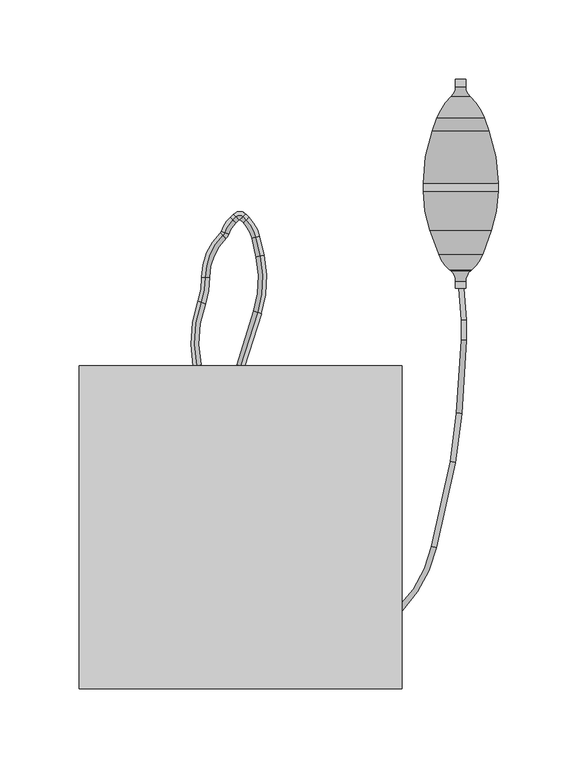
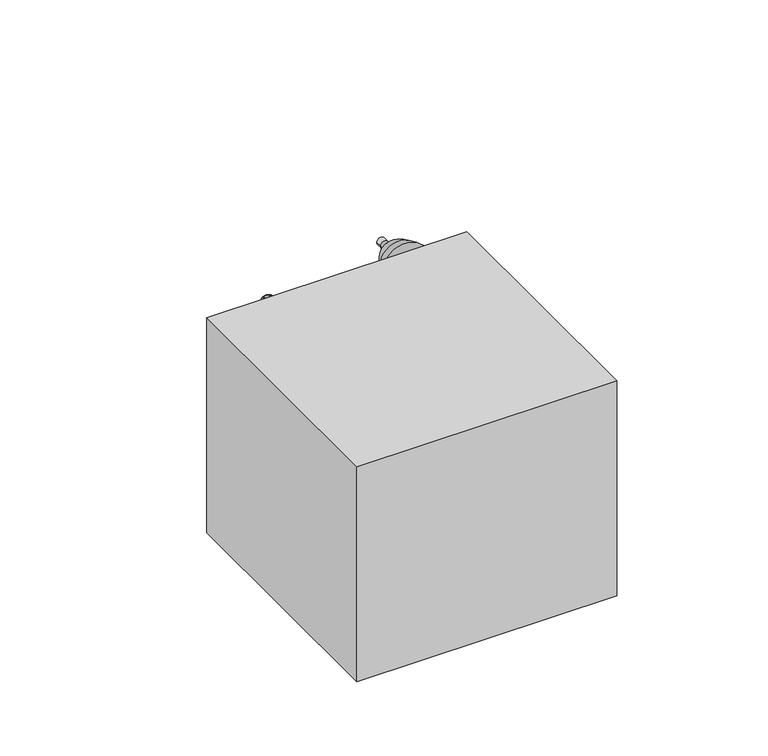
"""IFC4 building model written with IfcOpenShell, lengths in millimetres: proxy geometry, M4100 - Sphygmomanometer, Aneroid, Wall-Mounted : M4100 - Sphygmomanometer, Aneroid, Wall-Mounted."""

from ifc_helpers import new_model, si_unit, point, frame, frame_2d, origin, origin_with_axes, place, context, project, spatial, polyline, circle_curve, ellipse_curve, trimmed, segment, composite_curve, outline, extrude, source, transform, mapped, element, save
from ifc_brep_helpers import plane_surface, cylinder_surface, revolved_surface, extruded_surface, advanced_brep


def specialty_equipment_1a292596(model_context):
    return source(origin(), model_context, "Body", "SolidModel", [
        advanced_brep(
        [(0.0, 0.0, 93.3890108), (0.0, 0.0, 103.4609892), (10.60129, 33.4899695, 103.4609892), (10.60129, 33.4899695, 93.3890108), (12.1452256, 68.8519095, 103.4609892), (12.1452256, 68.8519095, 93.3890108), (9.4902706, 80.7634297, 103.4609892), (9.4902706, 80.7634297, 93.3890108), (3.5257448, 91.6206606, 103.4609892), (3.5257448, 91.6206606, 93.3890108), (1.489236, 93.6571694, 103.4609892), (1.489236, 93.6571694, 93.3890108), (-2.7411458, 93.6571694, 103.4609892), (-2.7411458, 93.6571694, 93.3890108), (-4.6658712, 91.732444, 103.4609892), (-4.6658712, 91.732444, 93.3890108), (-9.7582734, 83.8141156, 103.4609892), (-9.7582734, 83.8141156, 93.3890108), (-10.9708227, 81.9675873, 103.4609892), (-10.9708227, 81.9675873, 93.3890108), (-21.9594666, 55.7504476, 103.4609892), (-21.9594666, 55.7504476, 93.3890108), (-24.5939327, 39.9510684, 103.4609892), (-24.5939327, 39.9510684, 93.3890108), (-27.3580457, 0.1117834, 93.3890108), (-27.3580457, 0.1117834, 103.4609892)],
        [
            (0, 1, ellipse_curve(frame((0.0, 0.0, 98.425), z_axis=(-0.30179165133573443, -0.9533739031377199, 0.0), x_axis=(0.0, 0.0, 1.0)), 5.0359892, 2.5179946)),
            (1, 0, ellipse_curve(frame((0.0, 0.0, 98.425), z_axis=(-0.30179165133573443, -0.9533739031377199, 0.0), x_axis=(0.0, 0.0, 1.0)), 5.0359892, 2.5179946)),
            (1, 2),
            (2, 3, ellipse_curve(frame((10.60129, 33.4899695, 98.425), z_axis=(-0.3017916513357344, -0.9533739031377201, 0.0), x_axis=(0.0, 0.0, 1.0)), 5.0359892, 2.5179946)),
            (3, 0),
            (3, 2, ellipse_curve(frame((10.60129, 33.4899695, 98.425), z_axis=(-0.3017916513357344, -0.9533739031377201, 0.0), x_axis=(0.0, 0.0, 1.0)), 5.0359892, 2.5179946)),
            (4, 5, ellipse_curve(frame((12.1452256, 68.8519095, 98.425), z_axis=(0.21755123234481033, -0.9760489031320381, 0.0), x_axis=(0.0, 0.0, 1.0)), 5.0359892, 2.5179946)),
            (5, 3, circle_curve(frame((-54.3137244, 54.0388951, 93.3890108), z_axis=(0.0, 0.0, -1.0), x_axis=(0.9533739031377199, -0.3017916513357344, 0.0)), 68.0897748)),
            (2, 4, circle_curve(frame((-54.3137244, 54.0388951, 103.4609892), z_axis=(0.0, 0.0, 1.0), x_axis=(0.9533739031377199, -0.3017916513357344, 0.0)), 68.0897748)),
            (5, 4, ellipse_curve(frame((12.1452256, 68.8519095, 98.425), z_axis=(0.21755123234481044, -0.9760489031320381, 0.0), x_axis=(0.0, 0.0, 1.0)), 5.0359892, 2.5179946)),
            (4, 6),
            (6, 7, ellipse_curve(frame((9.4902706, 80.7634297, 98.425), z_axis=(0.21755123234481058, -0.9760489031320381, 0.0), x_axis=(0.0, 0.0, 1.0)), 5.0359892, 2.5179946)),
            (7, 5),
            (7, 6, ellipse_curve(frame((9.4902706, 80.7634297, 98.425), z_axis=(0.21755123234481058, -0.9760489031320381, 0.0), x_axis=(0.0, 0.0, 1.0)), 5.0359892, 2.5179946)),
            (8, 9, ellipse_curve(frame((3.5257448, 91.6206606, 98.425), z_axis=(0.7071067811865478, -0.7071067811865472, 0.0), x_axis=(0.0, 0.0, 1.0)), 5.0359892, 2.5179946)),
            (9, 7, circle_curve(frame((-12.1562786, 75.9386371, 93.3890108), z_axis=(0.0, 0.0, -1.0), x_axis=(0.9760489031320378, 0.21755123234481052, 0.0)), 22.1777302)),
            (6, 8, circle_curve(frame((-12.1562786, 75.9386371, 103.4609892), z_axis=(0.0, 0.0, 1.0), x_axis=(0.9760489031320378, 0.21755123234481052, 0.0)), 22.1777302)),
            (9, 8, ellipse_curve(frame((3.5257448, 91.6206606, 98.425), z_axis=(0.7071067811865477, -0.7071067811865474, 0.0), x_axis=(0.0, 0.0, 1.0)), 5.0359892, 2.5179946)),
            (8, 10),
            (10, 11, ellipse_curve(frame((1.489236, 93.6571694, 98.425), z_axis=(0.7071067811865424, -0.7071067811865528, 0.0), x_axis=(0.0, 0.0, 1.0)), 5.0359892, 2.5179946)),
            (11, 9),
            (11, 10, ellipse_curve(frame((1.489236, 93.6571694, 98.425), z_axis=(0.7071067811865424, -0.7071067811865528, 0.0), x_axis=(0.0, 0.0, 1.0)), 5.0359892, 2.5179946)),
            (12, 13, ellipse_curve(frame((-2.7411458, 93.6571694, 98.425), z_axis=(0.7071067811865475, 0.7071067811865477, 0.0), x_axis=(0.0, 0.0, 1.0)), 5.0359892, 2.5179946)),
            (13, 11, circle_curve(frame((-0.6259549, 91.5419785, 93.3890108), z_axis=(0.0, 0.0, -1.0), x_axis=(0.7071067811865528, 0.7071067811865424, 0.0)), 2.9913317)),
            (10, 12, circle_curve(frame((-0.6259549, 91.5419785, 103.4609892), z_axis=(0.0, 0.0, 1.0), x_axis=(0.7071067811865528, 0.7071067811865424, 0.0)), 2.9913317)),
            (13, 12, ellipse_curve(frame((-2.7411458, 93.6571694, 98.425), z_axis=(0.7071067811865426, 0.7071067811865526, 0.0), x_axis=(0.0, 0.0, 1.0)), 5.0359892, 2.5179946)),
            (12, 14),
            (14, 15, ellipse_curve(frame((-4.6658712, 91.732444, 98.425), z_axis=(0.7071067811865434, 0.7071067811865517, 0.0), x_axis=(0.0, 0.0, 1.0)), 5.0359892, 2.5179946)),
            (15, 13),
            (15, 14, ellipse_curve(frame((-4.6658712, 91.732444, 98.425), z_axis=(0.7071067811865434, 0.7071067811865517, 0.0), x_axis=(0.0, 0.0, 1.0)), 5.0359892, 2.5179946)),
            (16, 17, ellipse_curve(frame((-9.7582734, 83.8141156, 98.425), z_axis=(0.35006716200403615, 0.9367246031179283, 0.0), x_axis=(0.0, 0.0, 1.0)), 5.0359892, 2.5179946)),
            (17, 15, circle_curve(frame((11.0161522, 76.0504205, 93.3890108), z_axis=(0.0, 0.0, -1.0), x_axis=(-0.7071067811865517, 0.7071067811865434, 0.0)), 22.1777302)),
            (14, 16, circle_curve(frame((11.0161522, 76.0504205, 103.4609892), z_axis=(0.0, 0.0, 1.0), x_axis=(-0.7071067811865517, 0.7071067811865434, 0.0)), 22.1777302)),
            (17, 16, ellipse_curve(frame((-9.7582734, 83.8141156, 98.425), z_axis=(0.35006716200403576, 0.9367246031179283, 0.0), x_axis=(0.0, 0.0, 1.0)), 5.0359892, 2.5179946)),
            (18, 19, ellipse_curve(frame((-10.9708227, 81.9675873, 98.425), z_axis=(0.7204486556395683, 0.6935082801143322, 0.0), x_axis=(0.0, 0.0, 1.0)), 5.0359892, 2.5179946)),
            (19, 17, circle_curve(frame((-14.4282922, 85.5593673, 93.3890108), z_axis=(0.0, 0.0, 1.0), x_axis=(0.9367246031179312, -0.3500671620040279, 0.0)), 4.9854768)),
            (16, 18, circle_curve(frame((-14.4282922, 85.5593673, 103.4609892), z_axis=(0.0, 0.0, -1.0), x_axis=(0.9367246031179312, -0.3500671620040279, 0.0)), 4.9854768)),
            (19, 18, ellipse_curve(frame((-10.9708227, 81.9675873, 98.425), z_axis=(0.7204486556395688, 0.6935082801143314, 0.0), x_axis=(0.0, 0.0, 1.0)), 5.0359892, 2.5179946)),
            (20, 21, ellipse_curve(frame((-21.9594666, 55.7504476, 98.425), z_axis=(-0.010655908230738531, 0.9999432241981432, 0.0), x_axis=(0.0, 0.0, 1.0)), 5.0359892, 2.5179946)),
            (21, 19, circle_curve(frame((13.8981281, 56.1325645, 93.3890108), z_axis=(0.0, 0.0, -1.0), x_axis=(-0.6935082801143324, 0.7204486556395678, 0.0)), 35.8596307)),
            (18, 20, circle_curve(frame((13.8981281, 56.1325645, 103.4609892), z_axis=(0.0, 0.0, 1.0), x_axis=(-0.6935082801143324, 0.7204486556395678, 0.0)), 35.8596307)),
            (21, 20, ellipse_curve(frame((-21.9594666, 55.7504476, 98.425), z_axis=(-0.010655908230738309, 0.9999432241981432, 0.0), x_axis=(0.0, 0.0, 1.0)), 5.0359892, 2.5179946)),
            (22, 23, ellipse_curve(frame((-24.5939327, 39.9510684, 98.425), z_axis=(0.33452931398523156, 0.9423853447950952, 0.0), x_axis=(0.0, 0.0, 1.0)), 5.0359892, 2.5179946)),
            (23, 21, circle_curve(frame((-67.7275968, 55.2627189, 93.3890108), z_axis=(0.0, 0.0, 1.0), x_axis=(0.9999432241981431, 0.010655908230754234, 0.0)), 45.7707289)),
            (20, 22, circle_curve(frame((-67.7275968, 55.2627189, 103.4609892), z_axis=(0.0, 0.0, -1.0), x_axis=(0.9999432241981431, 0.010655908230754234, 0.0)), 45.7707289)),
            (23, 22, ellipse_curve(frame((-24.5939327, 39.9510684, 98.425), z_axis=(0.3345293139852315, 0.9423853447950952, 0.0), x_axis=(0.0, 0.0, 1.0)), 5.0359892, 2.5179946)),
            (24, 25, ellipse_curve(frame((-27.3580457, 0.1117834, 98.425), z_axis=(0.2011821163330489, -0.9795538556239548, 0.0), x_axis=(0.0, 0.0, 1.0)), 5.0359892, 2.5179946)),
            (25, 24, ellipse_curve(frame((-27.3580457, 0.1117834, 98.425), z_axis=(0.2011821163330489, -0.9795538556239548, 0.0), x_axis=(0.0, 0.0, 1.0)), 5.0359892, 2.5179946)),
            (24, 23, circle_curve(frame((45.4884963, 15.0731063, 93.3890108), z_axis=(0.0, 0.0, -1.0), x_axis=(-0.9423853447950952, 0.33452931398523145, 0.0)), 74.3670617)),
            (22, 25, circle_curve(frame((45.4884963, 15.0731063, 103.4609892), z_axis=(0.0, 0.0, 1.0), x_axis=(-0.9423853447950952, 0.33452931398523145, 0.0)), 74.3670617)),
        ],
        [
            plane_surface(frame((0.0, 0.0, 98.425), z_axis=(-0.30179165133573443, -0.9533739031377199, 0.0), x_axis=(0.0, 0.0, 1.0))),
            extruded_surface(trimmed(ellipse_curve(frame((0.0, 0.0, 98.425), z_axis=(0.30179165133573443, 0.9533739031377199, 0.0), x_axis=(0.0, 0.0, 1.0)), 5.0359892, 2.5179946), [point((0.0, 0.0, 93.3890108))], [point((0.0, 0.0, 103.4609892))], True, "CARTESIAN"), (10.60129, 33.4899695, 0.0), 35.1278437535672),
            extruded_surface(trimmed(ellipse_curve(frame((0.0, 0.0, 98.425), z_axis=(0.30179165133573443, 0.9533739031377199, 0.0), x_axis=(0.0, 0.0, 1.0)), 5.0359892, 2.5179946), [point((0.0, 0.0, 103.4609892))], [point((0.0, 0.0, 93.3890108))], True, "CARTESIAN"), (10.60129, 33.4899695, 0.0), 35.1278437535672),
            revolved_surface(trimmed(ellipse_curve(frame((10.60129, 33.4899695, 98.425), z_axis=(0.3017916513357343, 0.9533739031377199, 0.0), x_axis=(0.0, 0.0, 1.0)), 5.0359892, 2.5179946), [point((10.60129, 33.4899695, 93.3890108))], [point((10.60129, 33.4899695, 103.4609892))], True, "CARTESIAN"), (-54.3137244, 54.0388951, 98.425), (0.0, 0.0, -1.0)),
            revolved_surface(trimmed(ellipse_curve(frame((10.60129, 33.4899695, 98.425), z_axis=(0.3017916513357343, 0.9533739031377199, 0.0), x_axis=(0.0, 0.0, 1.0)), 5.0359892, 2.5179946), [point((10.60129, 33.4899695, 103.4609892))], [point((10.60129, 33.4899695, 93.3890108))], True, "CARTESIAN"), (-54.3137244, 54.0388951, 98.425), (0.0, 0.0, -1.0)),
            extruded_surface(trimmed(ellipse_curve(frame((12.1452256, 68.8519095, 98.425), z_axis=(-0.2175512323448103, 0.976048903132038, 0.0), x_axis=(0.0, 0.0, 1.0)), 5.0359892, 2.5179946), [point((12.1452256, 68.8519095, 93.3890108))], [point((12.1452256, 68.8519095, 103.4609892))], True, "CARTESIAN"), (-2.6549549999999993, 11.911520199999998, 0.0), 12.203814957915126),
            extruded_surface(trimmed(ellipse_curve(frame((12.1452256, 68.8519095, 98.425), z_axis=(-0.2175512323448103, 0.976048903132038, 0.0), x_axis=(0.0, 0.0, 1.0)), 5.0359892, 2.5179946), [point((12.1452256, 68.8519095, 103.4609892))], [point((12.1452256, 68.8519095, 93.3890108))], True, "CARTESIAN"), (-2.6549549999999993, 11.911520199999998, 0.0), 12.203814957915126),
            revolved_surface(trimmed(ellipse_curve(frame((9.4902706, 80.7634297, 98.425), z_axis=(-0.21755123234481052, 0.9760489031320378, 0.0), x_axis=(0.0, 0.0, 1.0)), 5.0359892, 2.5179946), [point((9.4902706, 80.7634297, 93.3890108))], [point((9.4902706, 80.7634297, 103.4609892))], True, "CARTESIAN"), (-12.1562786, 75.9386371, 98.425), (0.0, 0.0, -1.0)),
            revolved_surface(trimmed(ellipse_curve(frame((9.4902706, 80.7634297, 98.425), z_axis=(-0.21755123234481052, 0.9760489031320378, 0.0), x_axis=(0.0, 0.0, 1.0)), 5.0359892, 2.5179946), [point((9.4902706, 80.7634297, 103.4609892))], [point((9.4902706, 80.7634297, 93.3890108))], True, "CARTESIAN"), (-12.1562786, 75.9386371, 98.425), (0.0, 0.0, -1.0)),
            extruded_surface(trimmed(ellipse_curve(frame((3.5257448, 91.6206606, 98.425), z_axis=(-0.707106781186548, 0.707106781186547, 0.0), x_axis=(0.0, 0.0, 1.0)), 5.0359892, 2.5179946), [point((3.5257448, 91.6206606, 93.3890108))], [point((3.5257448, 91.6206606, 103.4609892))], True, "CARTESIAN"), (-2.0365088, 2.036508800000007, 0.0), 2.8800583648521623),
            extruded_surface(trimmed(ellipse_curve(frame((3.5257448, 91.6206606, 98.425), z_axis=(-0.707106781186548, 0.707106781186547, 0.0), x_axis=(0.0, 0.0, 1.0)), 5.0359892, 2.5179946), [point((3.5257448, 91.6206606, 103.4609892))], [point((3.5257448, 91.6206606, 93.3890108))], True, "CARTESIAN"), (-2.0365088, 2.036508800000007, 0.0), 2.8800583648521623),
            revolved_surface(trimmed(ellipse_curve(frame((1.489236, 93.6571694, 98.425), z_axis=(-0.7071067811865424, 0.7071067811865528, 0.0), x_axis=(0.0, 0.0, 1.0)), 5.0359892, 2.5179946), [point((1.489236, 93.6571694, 93.3890108))], [point((1.489236, 93.6571694, 103.4609892))], True, "CARTESIAN"), (-0.6259549, 91.5419785, 98.425), (0.0, 0.0, -1.0)),
            revolved_surface(trimmed(ellipse_curve(frame((1.489236, 93.6571694, 98.425), z_axis=(-0.7071067811865424, 0.7071067811865528, 0.0), x_axis=(0.0, 0.0, 1.0)), 5.0359892, 2.5179946), [point((1.489236, 93.6571694, 103.4609892))], [point((1.489236, 93.6571694, 93.3890108))], True, "CARTESIAN"), (-0.6259549, 91.5419785, 98.425), (0.0, 0.0, -1.0)),
            extruded_surface(trimmed(ellipse_curve(frame((-2.7411458, 93.6571694, 98.425), z_axis=(-0.707106781186542, -0.7071067811865531, 0.0), x_axis=(0.0, 0.0, 1.0)), 5.0359892, 2.5179946), [point((-2.7411458, 93.6571694, 93.3890108))], [point((-2.7411458, 93.6571694, 103.4609892))], True, "CARTESIAN"), (-1.9247253999999998, -1.9247253999999998, 0.0), 2.72197276452398),
            extruded_surface(trimmed(ellipse_curve(frame((-2.7411458, 93.6571694, 98.425), z_axis=(-0.707106781186542, -0.7071067811865531, 0.0), x_axis=(0.0, 0.0, 1.0)), 5.0359892, 2.5179946), [point((-2.7411458, 93.6571694, 103.4609892))], [point((-2.7411458, 93.6571694, 93.3890108))], True, "CARTESIAN"), (-1.9247253999999998, -1.9247253999999998, 0.0), 2.72197276452398),
            revolved_surface(trimmed(ellipse_curve(frame((-4.6658712, 91.732444, 98.425), z_axis=(-0.7071067811865434, -0.7071067811865517, 0.0), x_axis=(0.0, 0.0, 1.0)), 5.0359892, 2.5179946), [point((-4.6658712, 91.732444, 93.3890108))], [point((-4.6658712, 91.732444, 103.4609892))], True, "CARTESIAN"), (11.0161522, 76.0504205, 98.425), (0.0, 0.0, -1.0)),
            revolved_surface(trimmed(ellipse_curve(frame((-4.6658712, 91.732444, 98.425), z_axis=(-0.7071067811865434, -0.7071067811865517, 0.0), x_axis=(0.0, 0.0, 1.0)), 5.0359892, 2.5179946), [point((-4.6658712, 91.732444, 103.4609892))], [point((-4.6658712, 91.732444, 93.3890108))], True, "CARTESIAN"), (11.0161522, 76.0504205, 98.425), (0.0, 0.0, -1.0)),
            revolved_surface(trimmed(ellipse_curve(frame((-9.7582734, 83.8141156, 98.425), z_axis=(-0.350067162004028, -0.9367246031179312, 0.0), x_axis=(0.0, 0.0, 1.0)), 5.0359892, 2.5179946), [point((-9.7582734, 83.8141156, 93.3890108))], [point((-9.7582734, 83.8141156, 103.4609892))], True, "CARTESIAN"), (-14.4282922, 85.5593673, 98.425), (0.0, 0.0, 1.0)),
            revolved_surface(trimmed(ellipse_curve(frame((-9.7582734, 83.8141156, 98.425), z_axis=(-0.350067162004028, -0.9367246031179312, 0.0), x_axis=(0.0, 0.0, 1.0)), 5.0359892, 2.5179946), [point((-9.7582734, 83.8141156, 103.4609892))], [point((-9.7582734, 83.8141156, 93.3890108))], True, "CARTESIAN"), (-14.4282922, 85.5593673, 98.425), (0.0, 0.0, 1.0)),
            revolved_surface(trimmed(ellipse_curve(frame((-10.9708227, 81.9675873, 98.425), z_axis=(-0.7204486556395681, -0.6935082801143322, 0.0), x_axis=(0.0, 0.0, 1.0)), 5.0359892, 2.5179946), [point((-10.9708227, 81.9675873, 93.3890108))], [point((-10.9708227, 81.9675873, 103.4609892))], True, "CARTESIAN"), (13.8981281, 56.1325645, 98.425), (0.0, 0.0, -1.0)),
            revolved_surface(trimmed(ellipse_curve(frame((-10.9708227, 81.9675873, 98.425), z_axis=(-0.7204486556395681, -0.6935082801143322, 0.0), x_axis=(0.0, 0.0, 1.0)), 5.0359892, 2.5179946), [point((-10.9708227, 81.9675873, 103.4609892))], [point((-10.9708227, 81.9675873, 93.3890108))], True, "CARTESIAN"), (13.8981281, 56.1325645, 98.425), (0.0, 0.0, -1.0)),
            revolved_surface(trimmed(ellipse_curve(frame((-21.9594666, 55.7504476, 98.425), z_axis=(0.010655908230753961, -0.9999432241981431, 0.0), x_axis=(0.0, 0.0, 1.0)), 5.0359892, 2.5179946), [point((-21.9594666, 55.7504476, 93.3890108))], [point((-21.9594666, 55.7504476, 103.4609892))], True, "CARTESIAN"), (-67.7275968, 55.2627189, 98.425), (0.0, 0.0, 1.0)),
            revolved_surface(trimmed(ellipse_curve(frame((-21.9594666, 55.7504476, 98.425), z_axis=(0.010655908230753961, -0.9999432241981431, 0.0), x_axis=(0.0, 0.0, 1.0)), 5.0359892, 2.5179946), [point((-21.9594666, 55.7504476, 103.4609892))], [point((-21.9594666, 55.7504476, 93.3890108))], True, "CARTESIAN"), (-67.7275968, 55.2627189, 98.425), (0.0, 0.0, 1.0)),
            plane_surface(frame((-27.3580457, 0.1117834, 98.425), z_axis=(0.201182116333049, -0.9795538556239548, 0.0), x_axis=(0.0, 0.0, 1.0))),
            revolved_surface(trimmed(ellipse_curve(frame((-24.5939327, 39.9510684, 98.425), z_axis=(-0.3345293139852318, -0.9423853447950951, 0.0), x_axis=(0.0, 0.0, 1.0)), 5.0359892, 2.5179946), [point((-24.5939327, 39.9510684, 93.3890108))], [point((-24.5939327, 39.9510684, 103.4609892))], True, "CARTESIAN"), (45.4884963, 15.0731063, 98.425), (0.0, 0.0, -1.0)),
            revolved_surface(trimmed(ellipse_curve(frame((-24.5939327, 39.9510684, 98.425), z_axis=(-0.3345293139852318, -0.9423853447950951, 0.0), x_axis=(0.0, 0.0, 1.0)), 5.0359892, 2.5179946), [point((-24.5939327, 39.9510684, 103.4609892))], [point((-24.5939327, 39.9510684, 93.3890108))], True, "CARTESIAN"), (45.4884963, 15.0731063, 98.425), (0.0, 0.0, -1.0)),
        ],
        [
            (0, [[1, 2]]),
            (1, [[3, 4, 5, -2]]),
            (2, [[-5, 6, -3, -1]]),
            (3, [[7, 8, -4, 9]]),
            (4, [[10, -9, -6, -8]]),
            (5, [[11, 12, 13, -7]]),
            (6, [[-13, 14, -11, -10]]),
            (7, [[15, 16, -12, 17]]),
            (8, [[18, -17, -14, -16]]),
            (9, [[19, 20, 21, -15]]),
            (10, [[-21, 22, -19, -18]]),
            (11, [[23, 24, -20, 25]]),
            (12, [[26, -25, -22, -24]]),
            (13, [[27, 28, 29, -23]]),
            (14, [[-29, 30, -27, -26]]),
            (15, [[31, 32, -28, 33]]),
            (16, [[34, -33, -30, -32]]),
            (17, [[35, 36, -31, 37]]),
            (18, [[38, -37, -34, -36]]),
            (19, [[39, 40, -35, 41]]),
            (20, [[42, -41, -38, -40]]),
            (21, [[43, 44, -39, 45]]),
            (22, [[46, -45, -42, -44]]),
            (23, [[47, 48]]),
            (24, [[-47, 49, -43, 50]]),
            (25, [[-48, -50, -46, -49]]),
        ],
    ),
        advanced_brep(
        [(138.1282079, 48.8005767, 47.6946196), (135.3817713, 48.8005767, 47.6946196), (141.8571136, 48.8005767, 47.6946196), (139.110677, 48.8005767, 47.6946196), (138.1282079, 180.1855223, 47.6946196), (139.110677, 180.1855223, 47.6946196), (135.3817713, 180.1855223, 47.6946196), (141.8571136, 180.1855223, 47.6946196), (135.3817713, 175.5632852, 47.6946196), (141.8571136, 175.5632852, 47.6946196), (132.7169258, 169.4696535, 47.6946196), (144.5219592, 169.4696535, 47.6946196), (123.7575473, 155.9951928, 47.6946196), (153.4813376, 155.9951928, 47.6946196), (120.8482177, 148.0018755, 47.6946196), (156.3906672, 148.0018755, 47.6946196), (114.9866942, 114.7595239, 47.6946196), (162.2521907, 114.7595239, 47.6946196), (114.9866942, 109.7483973, 47.6946196), (162.2521907, 109.7483973, 47.6946196), (119.3165907, 85.1923341, 47.6946196), (157.9222942, 85.1923341, 47.6946196), (124.8056359, 70.1113063, 47.6946196), (152.433249, 70.1113063, 47.6946196), (131.6106524, 60.3927356, 47.6946196), (145.6282325, 60.3927356, 47.6946196), (132.2844617, 59.8273424, 47.6946196), (144.9544232, 59.8273424, 47.6946196), (135.3817713, 53.1851407, 47.6946196), (141.8571136, 53.1851407, 47.6946196)],
        [
            (0, 1),
            (1, 2, circle_curve(frame((138.6194425, 48.8005767, 47.6946196), z_axis=(0.0, -1.0, 0.0), x_axis=(1.0, 0.0, 0.0)), 3.2376712)),
            (2, 3),
            (3, 0, circle_curve(frame((138.6194425, 48.8005767, 47.6946196), z_axis=(0.0, 1.0, 0.0), x_axis=(1.0, 0.0, 0.0)), 0.4912345)),
            (2, 1, circle_curve(frame((138.6194425, 48.8005767, 47.6946196), z_axis=(0.0, -1.0, 0.0), x_axis=(1.0, 0.0, 0.0)), 3.2376712)),
            (0, 3, circle_curve(frame((138.6194425, 48.8005767, 47.6946196), z_axis=(0.0, 1.0, 0.0), x_axis=(1.0, 0.0, 0.0)), 0.4912345)),
            (4, 0),
            (3, 5),
            (5, 4, circle_curve(frame((138.6194425, 180.1855223, 47.6946196), z_axis=(0.0, 1.0, 0.0), x_axis=(1.0, 0.0, 0.0)), 0.4912345)),
            (4, 5, circle_curve(frame((138.6194425, 180.1855223, 47.6946196), z_axis=(0.0, 1.0, 0.0), x_axis=(1.0, 0.0, 0.0)), 0.4912345)),
            (6, 4),
            (5, 7),
            (7, 6, circle_curve(frame((138.6194425, 180.1855223, 47.6946196), z_axis=(0.0, 1.0, 0.0), x_axis=(1.0, 0.0, 0.0)), 3.2376712)),
            (6, 7, circle_curve(frame((138.6194425, 180.1855223, 47.6946196), z_axis=(0.0, 1.0, 0.0), x_axis=(1.0, 0.0, 0.0)), 3.2376712)),
            (8, 6),
            (7, 9),
            (9, 8, circle_curve(frame((138.6194425, 175.5632852, 47.6946196), z_axis=(0.0, 1.0, 0.0), x_axis=(1.0, 0.0, 0.0)), 3.2376712)),
            (8, 9, circle_curve(frame((138.6194425, 175.5632852, 47.6946196), z_axis=(0.0, 1.0, 0.0), x_axis=(1.0, 0.0, 0.0)), 3.2376712)),
            (10, 8, circle_curve(frame((127.0822753, 175.5632852, 47.6946196), z_axis=(0.0, 0.0, 1.0), x_axis=(-1.0, 0.0, 0.0)), 8.299496)),
            (9, 11, circle_curve(frame((150.1566096, 175.5632852, 47.6946196), z_axis=(0.0, 0.0, 1.0), x_axis=(1.0, 0.0, 0.0)), 8.299496)),
            (11, 10, circle_curve(frame((138.6194425, 169.4696535, 47.6946196), z_axis=(0.0, 1.0, 0.0), x_axis=(1.0, 0.0, 0.0)), 5.9025167)),
            (10, 11, circle_curve(frame((138.6194425, 169.4696535, 47.6946196), z_axis=(0.0, 1.0, 0.0), x_axis=(1.0, 0.0, 0.0)), 5.9025167)),
            (12, 10, circle_curve(frame((156.0419683, 144.2446246, 47.6946196), z_axis=(0.0, 0.0, -1.0), x_axis=(-1.0, 0.0, 0.0)), 34.3563632)),
            (11, 13, circle_curve(frame((121.1969167, 144.2446246, 47.6946196), z_axis=(0.0, 0.0, -1.0), x_axis=(1.0, 0.0, 0.0)), 34.3563632)),
            (13, 12, circle_curve(frame((138.6194425, 155.9951928, 47.6946196), z_axis=(0.0, 1.0, 0.0), x_axis=(1.0, 0.0, 0.0)), 14.8618952)),
            (12, 13, circle_curve(frame((138.6194425, 155.9951928, 47.6946196), z_axis=(0.0, 1.0, 0.0), x_axis=(1.0, 0.0, 0.0)), 14.8618952)),
            (14, 12),
            (13, 15),
            (15, 14, circle_curve(frame((138.6194425, 148.0018755, 47.6946196), z_axis=(0.0, 1.0, 0.0), x_axis=(1.0, 0.0, 0.0)), 17.7712248)),
            (14, 15, circle_curve(frame((138.6194425, 148.0018755, 47.6946196), z_axis=(0.0, 1.0, 0.0), x_axis=(1.0, 0.0, 0.0)), 17.7712248)),
            (16, 14, circle_curve(frame((212.1808279, 114.7595239, 47.6946196), z_axis=(0.0, 0.0, -1.0), x_axis=(-1.0, 0.0, 0.0)), 97.1941337)),
            (15, 17, circle_curve(frame((65.058057, 114.7595239, 47.6946196), z_axis=(0.0, 0.0, -1.0), x_axis=(1.0, 0.0, 0.0)), 97.1941337)),
            (17, 16, circle_curve(frame((138.6194425, 114.7595239, 47.6946196), z_axis=(0.0, 1.0, 0.0), x_axis=(1.0, 0.0, 0.0)), 23.6327482)),
            (16, 17, circle_curve(frame((138.6194425, 114.7595239, 47.6946196), z_axis=(0.0, 1.0, 0.0), x_axis=(1.0, 0.0, 0.0)), 23.6327482)),
            (18, 16),
            (17, 19),
            (19, 18, circle_curve(frame((138.6194425, 109.7483973, 47.6946196), z_axis=(0.0, 1.0, 0.0), x_axis=(1.0, 0.0, 0.0)), 23.6327482)),
            (18, 19, circle_curve(frame((138.6194425, 109.7483973, 47.6946196), z_axis=(0.0, 1.0, 0.0), x_axis=(1.0, 0.0, 0.0)), 23.6327482)),
            (20, 18, circle_curve(frame((186.7838197, 109.7483973, 47.6946196), z_axis=(0.0, 0.0, -1.0), x_axis=(-1.0, 0.0, 0.0)), 71.7971255)),
            (19, 21, circle_curve(frame((90.4550652, 109.7483973, 47.6946196), z_axis=(0.0, 0.0, -1.0), x_axis=(1.0, 0.0, 0.0)), 71.7971255)),
            (21, 20, circle_curve(frame((138.6194425, 85.1923341, 47.6946196), z_axis=(0.0, 1.0, 0.0), x_axis=(1.0, 0.0, 0.0)), 19.3028518)),
            (20, 21, circle_curve(frame((138.6194425, 85.1923341, 47.6946196), z_axis=(0.0, 1.0, 0.0), x_axis=(1.0, 0.0, 0.0)), 19.3028518)),
            (22, 20),
            (21, 23),
            (23, 22, circle_curve(frame((138.6194425, 70.1113063, 47.6946196), z_axis=(0.0, 1.0, 0.0), x_axis=(1.0, 0.0, 0.0)), 13.8138065)),
            (22, 23, circle_curve(frame((138.6194425, 70.1113063, 47.6946196), z_axis=(0.0, 1.0, 0.0), x_axis=(1.0, 0.0, 0.0)), 13.8138065)),
            (24, 22, circle_curve(frame((146.3432441, 77.9503546, 47.6946196), z_axis=(0.0, 0.0, -1.0), x_axis=(-1.0, 0.0, 0.0)), 22.9198439)),
            (23, 25, circle_curve(frame((130.8956408, 77.9503546, 47.6946196), z_axis=(0.0, 0.0, -1.0), x_axis=(1.0, 0.0, 0.0)), 22.9198439)),
            (25, 24, circle_curve(frame((138.6194425, 60.3927356, 47.6946196), z_axis=(0.0, 1.0, 0.0), x_axis=(1.0, 0.0, 0.0)), 7.00879)),
            (24, 25, circle_curve(frame((138.6194425, 60.3927356, 47.6946196), z_axis=(0.0, 1.0, 0.0), x_axis=(1.0, 0.0, 0.0)), 7.00879)),
            (26, 24),
            (25, 27),
            (27, 26, circle_curve(frame((138.6194425, 59.8273424, 47.6946196), z_axis=(0.0, 1.0, 0.0), x_axis=(1.0, 0.0, 0.0)), 6.3349807)),
            (26, 27, circle_curve(frame((138.6194425, 59.8273424, 47.6946196), z_axis=(0.0, 1.0, 0.0), x_axis=(1.0, 0.0, 0.0)), 6.3349807)),
            (28, 26, circle_curve(frame((126.7109927, 53.1851407, 47.6946196), z_axis=(0.0, 0.0, 1.0), x_axis=(-1.0, 0.0, 0.0)), 8.6707786)),
            (27, 29, circle_curve(frame((150.5278923, 53.1851407, 47.6946196), z_axis=(0.0, 0.0, 1.0), x_axis=(1.0, 0.0, 0.0)), 8.6707786)),
            (29, 28, circle_curve(frame((138.6194425, 53.1851407, 47.6946196), z_axis=(0.0, 1.0, 0.0), x_axis=(1.0, 0.0, 0.0)), 3.2376712)),
            (28, 29, circle_curve(frame((138.6194425, 53.1851407, 47.6946196), z_axis=(0.0, 1.0, 0.0), x_axis=(1.0, 0.0, 0.0)), 3.2376712)),
            (1, 28),
            (29, 2),
        ],
        [
            plane_surface(frame((138.6194425, 48.8005767, 47.6946196), z_axis=(0.0, -1.0, 0.0), x_axis=(1.0, 0.0, 0.0))),
            revolved_surface(polyline([(139.11067699999998, 48.8005767, 47.6946196), (139.11067699999998, 180.1855223, 47.6946196)]), (138.6194425, 48.8005767, 47.6946196), (0.0, -1.0, 0.0)),
            plane_surface(frame((138.6194425, 180.1855223, 47.6946196), z_axis=(0.0, 1.0, 0.0), x_axis=(1.0, 0.0, 0.0))),
            cylinder_surface(frame((138.6194425, 48.8005767, 47.6946196), z_axis=(0.0, -1.0, 0.0), x_axis=(1.0, 0.0, 0.0)), 3.2376712),
            revolved_surface(trimmed(ellipse_curve(frame((150.1566096, 175.5632852, 47.6946196), z_axis=(0.0, 0.0, 1.0), x_axis=(1.0, 0.0, 0.0)), 8.299496, 8.299496), [point((141.8571136, 175.5632852, 47.6946196))], [point((144.5219592, 169.4696535, 47.6946196))], True, "CARTESIAN"), (138.6194425, 48.8005767, 47.6946196), (0.0, -1.0, 0.0)),
            revolved_surface(trimmed(ellipse_curve(frame((121.1969167, 144.2446246, 47.6946196), z_axis=(0.0, 0.0, -1.0), x_axis=(1.0, 0.0, 0.0)), 34.3563632, 34.3563632), [point((144.5219592, 169.4696535, 47.6946196))], [point((153.4813376, 155.9951928, 47.6946196))], True, "CARTESIAN"), (138.6194425, 48.8005767, 47.6946196), (0.0, -1.0, 0.0)),
            revolved_surface(polyline([(153.4813376, 155.9951928, 47.6946196), (156.3906672, 148.0018755, 47.6946196)]), (138.6194425, 48.8005767, 47.6946196), (0.0, -1.0, 0.0)),
            revolved_surface(trimmed(ellipse_curve(frame((65.058057, 114.7595239, 47.6946196), z_axis=(0.0, 0.0, -1.0), x_axis=(1.0, 0.0, 0.0)), 97.1941337, 97.1941337), [point((156.3906672, 148.0018755, 47.6946196))], [point((162.2521907, 114.7595239, 47.6946196))], True, "CARTESIAN"), (138.6194425, 48.8005767, 47.6946196), (0.0, -1.0, 0.0)),
            cylinder_surface(frame((138.6194425, 48.8005767, 47.6946196), z_axis=(0.0, -1.0, 0.0), x_axis=(1.0, 0.0, 0.0)), 23.6327482),
            revolved_surface(trimmed(ellipse_curve(frame((90.4550652, 109.7483973, 47.6946196), z_axis=(0.0, 0.0, -1.0), x_axis=(1.0, 0.0, 0.0)), 71.7971255, 71.7971255), [point((162.2521907, 109.7483973, 47.6946196))], [point((157.9222942, 85.1923341, 47.6946196))], True, "CARTESIAN"), (138.6194425, 48.8005767, 47.6946196), (0.0, -1.0, 0.0)),
            revolved_surface(polyline([(157.9222942, 85.1923341, 47.6946196), (152.433249, 70.1113063, 47.6946196)]), (138.6194425, 48.8005767, 47.6946196), (0.0, -1.0, 0.0)),
            revolved_surface(trimmed(ellipse_curve(frame((130.8956408, 77.9503546, 47.6946196), z_axis=(0.0, 0.0, -1.0), x_axis=(1.0, 0.0, 0.0)), 22.9198439, 22.9198439), [point((152.433249, 70.1113063, 47.6946196))], [point((145.6282325, 60.3927356, 47.6946196))], True, "CARTESIAN"), (138.6194425, 48.8005767, 47.6946196), (0.0, -1.0, 0.0)),
            revolved_surface(polyline([(145.6282325, 60.3927356, 47.6946196), (144.9544232, 59.8273424, 47.6946196)]), (138.6194425, 48.8005767, 47.6946196), (0.0, -1.0, 0.0)),
            revolved_surface(trimmed(ellipse_curve(frame((150.5278923, 53.1851407, 47.6946196), z_axis=(0.0, 0.0, 1.0), x_axis=(1.0, 0.0, 0.0)), 8.6707786, 8.6707786), [point((144.9544232, 59.8273424, 47.6946196))], [point((141.8571136, 53.1851407, 47.6946196))], True, "CARTESIAN"), (138.6194425, 48.8005767, 47.6946196), (0.0, -1.0, 0.0)),
        ],
        [
            (0, [[1, 2, 3, 4]]),
            (0, [[-3, 5, -1, 6]]),
            (1, [[7, -4, 8, 9]]),
            (1, [[-8, -6, -7, 10]]),
            (2, [[11, -9, 12, 13]]),
            (2, [[-12, -10, -11, 14]]),
            (3, [[15, -13, 16, 17]]),
            (3, [[-16, -14, -15, 18]]),
            (4, [[19, -17, 20, 21]]),
            (4, [[-20, -18, -19, 22]]),
            (5, [[23, -21, 24, 25]]),
            (5, [[-24, -22, -23, 26]]),
            (6, [[27, -25, 28, 29]]),
            (6, [[-28, -26, -27, 30]]),
            (7, [[31, -29, 32, 33]]),
            (7, [[-32, -30, -31, 34]]),
            (8, [[35, -33, 36, 37]]),
            (8, [[-36, -34, -35, 38]]),
            (9, [[39, -37, 40, 41]]),
            (9, [[-40, -38, -39, 42]]),
            (10, [[43, -41, 44, 45]]),
            (10, [[-44, -42, -43, 46]]),
            (11, [[47, -45, 48, 49]]),
            (11, [[-48, -46, -47, 50]]),
            (12, [[51, -49, 52, 53]]),
            (12, [[-52, -50, -51, 54]]),
            (13, [[55, -53, 56, 57]]),
            (13, [[-56, -54, -55, 58]]),
            (3, [[59, -57, 60, -2]]),
            (3, [[-60, -58, -59, -5]]),
        ],
    ),
        extrude(outline(composite_curve([segment(polyline([(60.0140495, 56.9161892), (60.0140495, -51.3523862)]), True, "CONTINUOUS"), segment(trimmed(circle_curve(frame_2d((49.7730325, -51.3523862)), 10.2410171), [point((60.0140495, -51.3523862))], [point((49.7730325, -61.5934033))], False, "CARTESIAN"), True, "CONTINUOUS"), segment(polyline([(49.7730325, -61.5934033), (47.625, -61.5934033)]), True, "CONTINUOUS"), segment(trimmed(circle_curve(frame_2d((47.625, -55.2434033)), 6.35), [point((47.625, -61.5934033))], [point((41.275, -55.2434033))], False, "CARTESIAN"), True, "CONTINUOUS"), segment(polyline([(41.275, -55.2434033), (41.275, 56.9161892)]), True, "CONTINUOUS"), segment(trimmed(circle_curve(frame_2d((47.625, 56.9161892)), 6.35), [point((41.275, 56.9161892))], [point((47.625, 63.2661892))], False, "CARTESIAN"), True, "CONTINUOUS"), segment(polyline([(47.625, 63.2661892), (53.6640495, 63.2661892)]), True, "CONTINUOUS"), segment(trimmed(circle_curve(frame_2d((53.6640495, 56.9161892)), 6.35), [point((53.6640495, 63.2661892))], [point((60.0140495, 56.9161892))], False, "CARTESIAN"), True, "CONTINUOUS")], self_intersect=False)), frame((0.0, -184.15, 0.0), z_axis=(0.0, 1.0, 0.0), x_axis=(0.0, 0.0, 1.0)), (0.0, 0.0, 1.0), 49.3242444),
        extrude(outline(polyline([(1.4455759, -86.4782162), (-0.7959523, -86.4782162), (0.3248118, -26.9185099), (1.4455759, -86.4782162)])), frame((0.0, 0.0, 98.425), z_axis=(0.0, 0.0, 1.0), x_axis=(1.0, 0.0, 0.0)), (0.0, 0.0, 1.0), 1.5875),
        advanced_brep(
        [(64.1302409, -157.2064783, 47.6946196), (63.006649, -160.2935217, 47.6946196), (78.2964296, -165.8585468, 47.6946196), (79.4200216, -162.7715033, 47.6946196), (93.3436181, -162.5226654, 47.6946196), (91.020657, -160.1997043, 47.6946196), (101.7868533, -154.0794302, 47.6946196), (99.4638922, -151.7564691, 47.6946196), (123.3936687, -114.6421744, 47.6946196), (120.1855696, -113.9347877, 47.6946196), (135.2214894, -61.0013237, 47.6946196), (132.0133902, -60.2939371, 47.6946196), (139.2461165, -30.2081991, 47.6946196), (135.9885723, -29.7831085, 47.6946196), (142.2495065, 16.0179543, 47.6946196), (138.9643435, 16.0179543, 47.6946196), (142.2495065, 28.7184587, 47.6946196), (138.9643435, 28.7184587, 47.6946196), (137.4726358, 48.678532, 47.6946196), (140.7487182, 48.9226214, 47.6946196)],
        [
            (0, 1, circle_curve(frame((63.568445, -158.75, 47.6946196), z_axis=(-0.9396926207859115, 0.3420201433256602, 0.0), x_axis=(-0.3420201433256602, -0.9396926207859115, 0.0)), 1.6425815)),
            (1, 0, circle_curve(frame((63.568445, -158.75, 47.6946196), z_axis=(-0.9396926207859115, 0.3420201433256602, 0.0), x_axis=(-0.3420201433256602, -0.9396926207859115, 0.0)), 1.6425815)),
            (1, 2),
            (2, 3, circle_curve(frame((78.8582256, -164.315025, 47.6946196), z_axis=(-0.9396926207859115, 0.3420201433256602, 0.0), x_axis=(-0.3420201433256602, -0.9396926207859115, 0.0)), 1.6425815)),
            (3, 0),
            (3, 2, circle_curve(frame((78.8582256, -164.315025, 47.6946196), z_axis=(-0.9396926207859115, 0.3420201433256602, 0.0), x_axis=(-0.3420201433256602, -0.9396926207859115, 0.0)), 1.6425815)),
            (4, 5, circle_curve(frame((92.1821375, -161.3611849, 47.6946196), z_axis=(-0.7071067811865444, -0.7071067811865509, 0.0), x_axis=(0.7071067811865509, -0.7071067811865444, 0.0)), 1.6425815)),
            (5, 3, circle_curve(frame((83.2018814, -152.3809287, 47.6946196), z_axis=(0.0, 0.0, -1.0), x_axis=(-0.34202014332565955, -0.9396926207859118, 0.0)), 11.0574185)),
            (2, 4, circle_curve(frame((83.2018814, -152.3809287, 47.6946196), z_axis=(0.0, 0.0, 1.0), x_axis=(-0.34202014332565955, -0.9396926207859118, 0.0)), 14.3425815)),
            (5, 4, circle_curve(frame((92.1821375, -161.3611849, 47.6946196), z_axis=(-0.707106781186547, -0.7071067811865481, 0.0), x_axis=(0.7071067811865481, -0.707106781186547, 0.0)), 1.6425815)),
            (4, 6),
            (6, 7, circle_curve(frame((100.6253728, -152.9179497, 47.6946196), z_axis=(-0.7071067811865462, -0.7071067811865489, 0.0), x_axis=(0.7071067811865489, -0.7071067811865462, 0.0)), 1.6425815)),
            (7, 5),
            (7, 6, circle_curve(frame((100.6253728, -152.9179497, 47.6946196), z_axis=(-0.7071067811865462, -0.7071067811865489, 0.0), x_axis=(0.7071067811865489, -0.7071067811865462, 0.0)), 1.6425815)),
            (8, 9, circle_curve(frame((121.7896192, -114.2884811, 47.6946196), z_axis=(-0.21532771486204566, -0.9765418450902602, 0.0), x_axis=(0.9765418450902602, -0.21532771486204566, 0.0)), 1.6425815)),
            (9, 7, circle_curve(frame((45.0818146, -97.3743915, 47.6946196), z_axis=(0.0, 0.0, -1.0), x_axis=(0.7071067811865482, -0.7071067811865469, 0.0)), 76.9078718)),
            (6, 8, circle_curve(frame((45.0818146, -97.3743915, 47.6946196), z_axis=(0.0, 0.0, 1.0), x_axis=(0.7071067811865482, -0.7071067811865469, 0.0)), 80.1930348)),
            (9, 8, circle_curve(frame((121.7896192, -114.2884811, 47.6946196), z_axis=(-0.21532771486204544, -0.9765418450902602, 0.0), x_axis=(0.9765418450902602, -0.21532771486204544, 0.0)), 1.6425815)),
            (8, 10),
            (10, 11, circle_curve(frame((133.6174398, -60.6476304, 47.6946196), z_axis=(-0.21532771486204544, -0.9765418450902602, 0.0), x_axis=(0.9765418450902602, -0.21532771486204544, 0.0)), 1.6425815)),
            (11, 9),
            (11, 10, circle_curve(frame((133.6174398, -60.6476304, 47.6946196), z_axis=(-0.21532771486204544, -0.9765418450902602, 0.0), x_axis=(0.9765418450902602, -0.21532771486204544, 0.0)), 1.6425815)),
            (10, 12),
            (12, 13, circle_curve(frame((137.6173444, -29.9956538, 47.6946196), z_axis=(-0.12939709806477467, -0.9915928554666049, 0.0), x_axis=(0.9915928554666049, -0.12939709806477467, 0.0)), 1.6425815)),
            (13, 11),
            (13, 12, circle_curve(frame((137.6173444, -29.9956538, 47.6946196), z_axis=(-0.12939709806477467, -0.9915928554666049, 0.0), x_axis=(0.9915928554666049, -0.12939709806477467, 0.0)), 1.6425815)),
            (14, 15, circle_curve(frame((140.606925, 16.0179543, 47.6946196), z_axis=(0.0, -1.0, 0.0), x_axis=(1.0, 0.0, 0.0)), 1.6425815)),
            (15, 13, circle_curve(frame((-214.993075, 16.0179543, 47.6946196), z_axis=(0.0, 0.0, -1.0), x_axis=(0.9915928554666049, -0.12939709806477429, 0.0)), 353.9574185)),
            (12, 14, circle_curve(frame((-214.993075, 16.0179543, 47.6946196), z_axis=(0.0, 0.0, 1.0), x_axis=(0.9915928554666049, -0.12939709806477429, 0.0)), 357.2425815)),
            (15, 14, circle_curve(frame((140.606925, 16.0179543, 47.6946196), z_axis=(0.0, -1.0, 0.0), x_axis=(1.0, 0.0, 0.0)), 1.6425815)),
            (14, 16),
            (16, 17, circle_curve(frame((140.606925, 28.7184587, 47.6946196), z_axis=(0.0, -1.0, 0.0), x_axis=(1.0, 0.0, 0.0)), 1.6425815)),
            (17, 15),
            (17, 16, circle_curve(frame((140.606925, 28.7184587, 47.6946196), z_axis=(0.0, -1.0, 0.0), x_axis=(1.0, 0.0, 0.0)), 1.6425815)),
            (18, 19, circle_curve(frame((139.110677, 48.8005767, 47.6946196), z_axis=(-0.07430053978067924, 0.9972358947552479, 0.0), x_axis=(0.9972358947552479, 0.07430053978067924, 0.0)), 1.6425815)),
            (19, 18, circle_curve(frame((139.110677, 48.8005767, 47.6946196), z_axis=(-0.07430053978067924, 0.9972358947552479, 0.0), x_axis=(0.9972358947552479, 0.07430053978067924, 0.0)), 1.6425815)),
            (16, 19),
            (18, 17),
        ],
        [
            plane_surface(frame((63.568445, -158.75, 98.425), z_axis=(-0.9396926207859115, 0.3420201433256602, 0.0), x_axis=(0.0, 0.0, 1.0))),
            cylinder_surface(frame((63.568445, -158.75, 47.6946196), z_axis=(-0.9396926207859115, 0.3420201433256602, 0.0), x_axis=(-0.3420201433256602, -0.9396926207859115, 0.0)), 1.6425815),
            revolved_surface(trimmed(ellipse_curve(frame((78.8582256, -164.315025, 47.6946196), z_axis=(0.9396926207859118, -0.3420201433256596, 0.0), x_axis=(-0.3420201433256596, -0.9396926207859118, 0.0)), 1.6425815, 1.6425815), [point((79.4200216, -162.7715033, 47.6946196))], [point((78.2964296, -165.8585468, 47.6946196))], True, "CARTESIAN"), (83.2018814, -152.3809287, 98.425), (0.0, 0.0, -1.0)),
            revolved_surface(trimmed(ellipse_curve(frame((78.8582256, -164.315025, 47.6946196), z_axis=(0.9396926207859118, -0.3420201433256596, 0.0), x_axis=(-0.3420201433256596, -0.9396926207859118, 0.0)), 1.6425815, 1.6425815), [point((78.2964296, -165.8585468, 47.6946196))], [point((79.4200216, -162.7715033, 47.6946196))], True, "CARTESIAN"), (83.2018814, -152.3809287, 98.425), (0.0, 0.0, -1.0)),
            cylinder_surface(frame((92.1821375, -161.3611849, 47.6946196), z_axis=(-0.7071067811865462, -0.7071067811865489, 0.0), x_axis=(0.7071067811865489, -0.7071067811865462, 0.0)), 1.6425815),
            revolved_surface(trimmed(ellipse_curve(frame((100.6253728, -152.9179497, 47.6946196), z_axis=(0.707106781186547, 0.7071067811865481, 0.0), x_axis=(0.7071067811865481, -0.707106781186547, 0.0)), 1.6425815, 1.6425815), [point((99.4638922, -151.7564691, 47.6946196))], [point((101.7868533, -154.0794302, 47.6946196))], True, "CARTESIAN"), (45.0818146, -97.3743915, 98.425), (0.0, 0.0, -1.0)),
            revolved_surface(trimmed(ellipse_curve(frame((100.6253728, -152.9179497, 47.6946196), z_axis=(0.707106781186547, 0.7071067811865481, 0.0), x_axis=(0.7071067811865481, -0.707106781186547, 0.0)), 1.6425815, 1.6425815), [point((101.7868533, -154.0794302, 47.6946196))], [point((99.4638922, -151.7564691, 47.6946196))], True, "CARTESIAN"), (45.0818146, -97.3743915, 98.425), (0.0, 0.0, -1.0)),
            cylinder_surface(frame((121.7896192, -114.2884811, 47.6946196), z_axis=(-0.21532771486204544, -0.9765418450902602, 0.0), x_axis=(0.9765418450902602, -0.21532771486204544, 0.0)), 1.6425815),
            cylinder_surface(frame((133.6174398, -60.6476304, 47.6946196), z_axis=(-0.12939709806477467, -0.9915928554666049, 0.0), x_axis=(0.9915928554666049, -0.12939709806477467, 0.0)), 1.6425815),
            revolved_surface(trimmed(ellipse_curve(frame((137.6173444, -29.9956538, 47.6946196), z_axis=(0.1293970980647746, 0.9915928554666049, 0.0), x_axis=(0.9915928554666049, -0.1293970980647746, 0.0)), 1.6425815, 1.6425815), [point((135.9885723, -29.7831085, 47.6946196))], [point((139.2461165, -30.2081991, 47.6946196))], True, "CARTESIAN"), (-214.993075, 16.0179543, 98.425), (0.0, 0.0, -1.0)),
            revolved_surface(trimmed(ellipse_curve(frame((137.6173444, -29.9956538, 47.6946196), z_axis=(0.1293970980647746, 0.9915928554666049, 0.0), x_axis=(0.9915928554666049, -0.1293970980647746, 0.0)), 1.6425815, 1.6425815), [point((139.2461165, -30.2081991, 47.6946196))], [point((135.9885723, -29.7831085, 47.6946196))], True, "CARTESIAN"), (-214.993075, 16.0179543, 98.425), (0.0, 0.0, -1.0)),
            cylinder_surface(frame((140.606925, 16.0179543, 47.6946196), z_axis=(0.0, -1.0, 0.0), x_axis=(1.0, 0.0, 0.0)), 1.6425815),
            plane_surface(frame((139.110677, 48.8005767, 98.425), z_axis=(-0.07430053978067952, 0.9972358947552479, 0.0), x_axis=(0.0, 0.0, 1.0))),
            cylinder_surface(frame((140.606925, 28.7184587, 47.6946196), z_axis=(0.07430053978067924, -0.9972358947552479, 0.0), x_axis=(0.9972358947552479, 0.07430053978067924, 0.0)), 1.6425815),
        ],
        [
            (0, [[1, 2]]),
            (1, [[3, 4, 5, -2]]),
            (1, [[-5, 6, -3, -1]]),
            (2, [[7, 8, -4, 9]]),
            (3, [[10, -9, -6, -8]]),
            (4, [[11, 12, 13, -7]]),
            (4, [[-13, 14, -11, -10]]),
            (5, [[15, 16, -12, 17]]),
            (6, [[18, -17, -14, -16]]),
            (7, [[19, 20, 21, -15]]),
            (7, [[-21, 22, -19, -18]]),
            (8, [[23, 24, 25, -20]]),
            (8, [[-25, 26, -23, -22]]),
            (9, [[27, 28, -24, 29]]),
            (10, [[30, -29, -26, -28]]),
            (11, [[31, 32, 33, -27]]),
            (11, [[-33, 34, -31, -30]]),
            (12, [[35, 36]]),
            (13, [[37, -35, 38, -32]]),
            (13, [[-38, -36, -37, -34]]),
        ],
    ),
        extrude(outline(composite_curve([segment(trimmed(circle_curve(frame_2d((-142.2191525, 42.6389159)), 25.4), [point((-120.2221073, 29.9389159))], [point((-118.3509599, 51.3262276))], True, "CARTESIAN"), True, "CONTINUOUS"), segment(polyline([(-118.3509599, 51.3262276), (-125.0930617, 69.85), (-69.85, 69.85), (-78.1567361, 47.0274301)]), True, "CONTINUOUS"), segment(trimmed(circle_curve(frame_2d((-38.3859034, 32.5520308)), 42.3232361), [point((-78.1567361, 47.0274301))], [point((-80.7091396, 32.5520308))], True, "CARTESIAN"), True, "CONTINUOUS"), segment(polyline([(-80.7091396, 32.5520308), (-80.7091396, 12.7), (-130.175, 12.7), (-120.2221073, 29.9389159)]), True, "CONTINUOUS")], self_intersect=False)), frame((-19.05, 0.0, 0.0), z_axis=(1.0, 0.0, 0.0), x_axis=(0.0, 1.0, 0.0)), (0.0, 0.0, 1.0), 38.1),
        extrude(outline(polyline([(44.45, -142.875), (-44.45, -142.875), (-44.45, -53.975), (44.45, -53.975), (44.45, -142.875)])), origin_with_axes(), (0.0, 0.0, 1.0), 12.7),
        extrude(outline(polyline([(79.375, -158.75), (-79.375, -158.75), (-79.375, 0.0), (79.375, 0.0), (79.375, -158.75)]), holes=[polyline([(76.2, -155.575), (76.2, -3.175), (-76.2, -3.175), (-76.2, -155.575), (76.2, -155.575)])]), frame((0.0, 0.0, 95.25), z_axis=(0.0, 0.0, 1.0), x_axis=(1.0, 0.0, 0.0)), (0.0, 0.0, 1.0), 6.35),
        extrude(outline(polyline([(79.375, 0.0), (79.375, -158.75), (-79.375, -158.75), (-79.375, 0.0), (79.375, 0.0)])), frame((0.0, 0.0, 69.85), z_axis=(0.0, 0.0, 1.0), x_axis=(1.0, 0.0, 0.0)), (0.0, 0.0, 1.0), 25.4),
        extrude(outline(polyline([(101.6, -203.2), (-101.6, -203.2), (-101.6, 0.0), (101.6, 0.0), (101.6, -203.2)])), origin_with_axes(), (0.0, 0.0, 1.0), 177.8),
    ])


if __name__ == "__main__":
    model = new_model("IFC4")
    model_context = context("Model", 3, world=origin())
    ifc_project = project(units=[si_unit("LENGTHUNIT", "METRE", prefix="MILLI")], contexts=[model_context])
    site = spatial("IfcSite", under=ifc_project)
    building = spatial("IfcBuilding", under=site)
    placement = place(None, origin())
    specialty_equipment_shape = specialty_equipment_1a292596(model_context)
    element("IfcBuildingElementProxy", 1, Name="M4100 - Sphygmomanometer, Aneroid, Wall-Mounted : M4100 - Sphygmomanometer, Aneroid, Wall-Mounted", ObjectType="M4100 - Sphygmomanometer, Aneroid, Wall-Mounted : M4100 - Sphygmomanometer, Aneroid, Wall-Mounted", at=placement, inside=building, context=model_context, shape_type="MappedRepresentation", body=[
        mapped(specialty_equipment_shape, transform((0.0, 0.0, 0.0), x_axis=(1.0, 0.0, 0.0), y_axis=(0.0, 1.0, 0.0), z_axis=(0.0, 0.0, 1.0))),
    ])
    save(model, "model.ifc")

# Revit data of these elements
# Project information
#   Room Abbreviation = "BRII2/BRAR2"
#   Room Description 3-1 = "Bedroom, ICU/CCU, Protective Environment (BRII2)"
#   Room Description 3-2 = "Anteroom, Protective Environment (BRAR2)"
#   Room Description 3-3 = "Toilet/Shower (TLTS2)"
#   Sheets - Total = "9"
#   Project Issue Date = "Issue Date"
#   Project Status = "Project Status"
#   Client Name = "Owner"
#   Project Address = "Enter address here"
#   Project Name = "Project Name"
#   Project Number = "Project Number"
#   Publication Date = "1-Feb-16"
# Type "M4100 - Sphygmomanometer, Aneroid, Wall-Mounted : M4100 - Sphygmomanometer, Aneroid, Wall-Mounted"
#   Watts2 = "0"
#   Watts1 = "0"
#   Unit_Issue = "EA"
#   UTIL_6_Misc = "-"
#   UTIL_5_NonMedGas = "-"
#   UTIL_4_MiscGas = "-"
#   UTIL_3_MedGas = "-"
#   UTIL_2_Elec = "-"
#   UTIL_1_WaterDrain = "-"
#   Nomenclature = "Sphygmomanometer, Aneroid, Wall Mounted"
#   NSN = "6520"
#   Location [instance default] = ""
#   JSN = "M4100"
#   Fund_Source_VA = "-"
#   Fund_Source_Navy = "-"
#   Fund_Source_Army = "-"
#   Fund_Source_AF = "-"
#   ELEC_Volts2 = "0"
#   ELEC_Volts1 = "0"
#   ELEC_Phase2 = "0"
#   ELEC_Phase1 = "0"
#   ELEC_HertzSwitch = "0"
#   ELEC_HertzDependent = "0"
#   ELEC_Hertz = "0"
#   ELEC_Amps2 = "0"
#   ELEC_Amps1 = "0"
#   DetailDescription = "Aneroid sphygmomanometer. Unit is wall mounted and has large graphic dial display for easy reading from all angles. It has a 90 degree (angle) swivel and 10 degree (angle) forward tilt to reduce glare. Unit accuracy is within 1% of reading. Sturdy impact-resistant construction."
#   CAT_VA = "C"
#   CAT_Navy = "C"
#   CAT_IHS = "-"
#   CAT_Army = "C"
#   CAT_AF = "C"
#   BTUperhour = "0"
#   mounting height [instance default] = 0' - 0"
#   Weight_IP = 5
#   Default Elevation = 4' - 0"
#   DIM_Width_IP = 0' - 8"
#   DIM_Height_IP = 0' - 8"
#   DIM_Depth_IP = 0' - 7"
#   finish [instance default] = none
#   Assembly Code = ""
# Element 1 (IfcBuildingElementProxy, "M4100 - Sphygmomanometer, Aneroid, Wall-Mounted : M4100 - Sphygmomanometer, Aneroid, Wall-Mounted")
#   Location = "BRII2"
#   Materials on its faces: "EquipSpace"
# Materials
#   "EquipSpace": class "Unassigned", colour RGB 221 217 195, transparency 0.5
